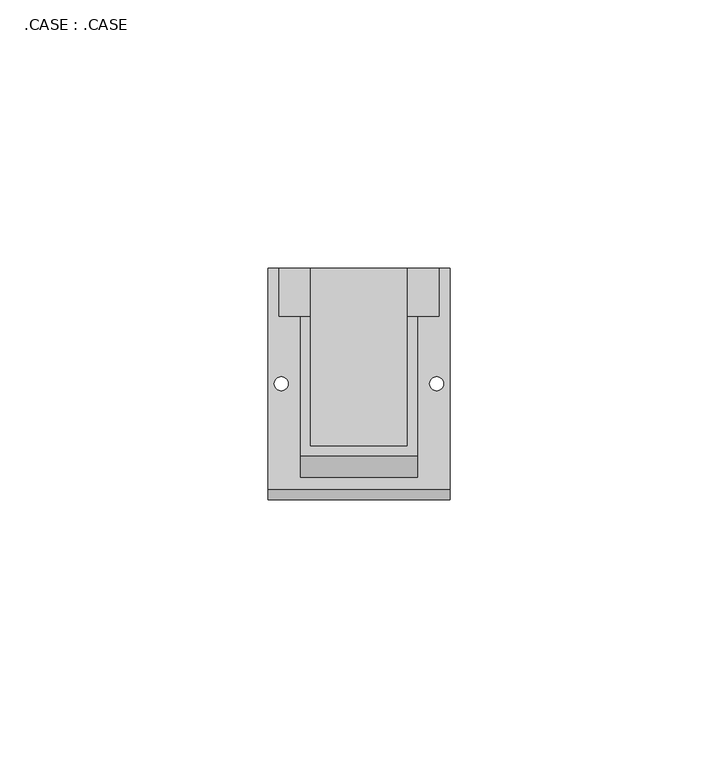
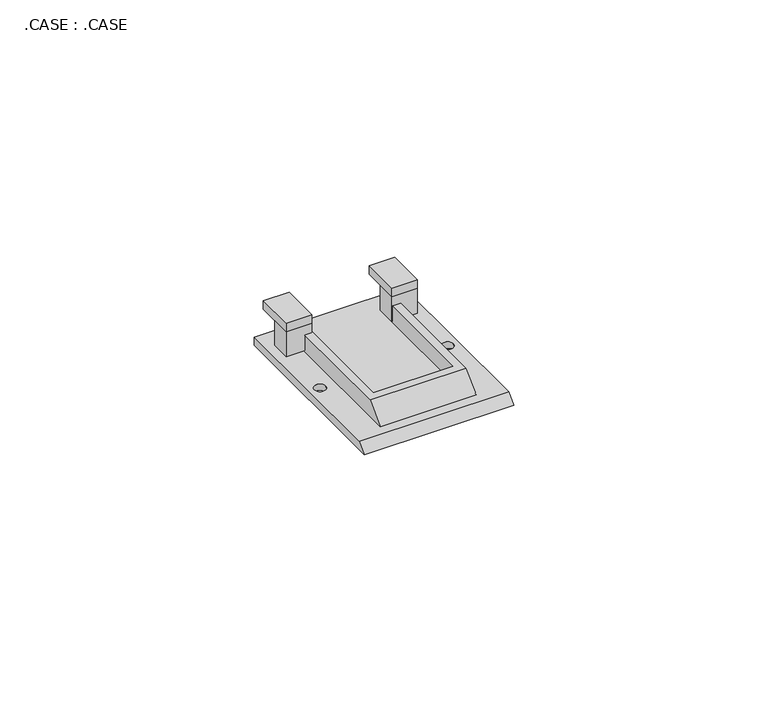
"""IFC4 building model written with IfcOpenShell, lengths in millimetres: proxy geometry, .CASE : .CASE."""

from ifc_helpers import new_model, si_unit, frame, origin, place, context, project, spatial, polyline, circle_curve, outline, extrude, source, transform, mapped, element, save
from ifc_brep_helpers import plane_surface, revolved_surface, advanced_brep


def case_case_fa127987(model_context):
    return source(origin(), model_context, "Body", "SolidModel", [
        extrude(outline(polyline([(1442.9350176, 13234.6739696), (1442.9350176, 13225.7186096), (1437.1350176, 13225.7186096), (1437.1350176, 13234.6739696), (1442.9350176, 13234.6739696)])), frame((0.0, 0.0, 8.0), z_axis=(0.0, 0.0, 1.0), x_axis=(1.0, 0.0, 0.0)), (0.0, 0.0, 1.0), 2.0),
        extrude(outline(polyline([(1461.1150176, 13234.6739696), (1466.9150176, 13234.6739696), (1466.9150176, 13225.7186096), (1461.1150176, 13225.7186096), (1461.1150176, 13234.6739696)])), frame((0.0, 0.0, 8.0), z_axis=(0.0, 0.0, 1.0), x_axis=(1.0, 0.0, 0.0)), (0.0, 0.0, 1.0), 2.0),
        extrude(outline(polyline([(1442.9350176, 13230.2186096), (1442.9350176, 13225.7186096), (1437.1350176, 13225.7186096), (1437.1350176, 13230.2186096), (1442.9350176, 13230.2186096)])), frame((0.0, 0.0, 2.0), z_axis=(0.0, 0.0, 1.0), x_axis=(1.0, 0.0, 0.0)), (0.0, 0.0, 1.0), 6.0),
        extrude(outline(polyline([(1461.1150176, 13230.2186096), (1466.9150176, 13230.2186096), (1466.9150176, 13225.7186096), (1461.1150176, 13225.7186096), (1461.1150176, 13230.2186096)])), frame((0.0, 0.0, 2.0), z_axis=(0.0, 0.0, 1.0), x_axis=(1.0, 0.0, 0.0)), (0.0, 0.0, 1.0), 6.0),
        advanced_brep(
        [(1469.0250176, 13193.4256546, 2.0), (1469.0250176, 13234.6739696, 2.0), (1435.0250176, 13234.6739696, 2.0), (1435.0250176, 13193.4256546, 2.0), (1441.1350176, 13195.6739696, 2.0), (1441.1350176, 13225.7186096, 2.0), (1442.9350176, 13225.7186096, 2.0), (1442.9350176, 13201.4739696, 2.0), (1461.1150176, 13201.4739696, 2.0), (1461.1150176, 13225.7186096, 2.0), (1462.9150176, 13225.7186096, 2.0), (1462.9150176, 13195.6739696, 2.0), (1467.8250176, 13213.1041412, 2.0), (1465.2250176, 13213.1041412, 2.0), (1438.8250176, 13213.1041412, 2.0), (1436.2250176, 13213.1041412, 2.0), (1435.0250176, 13234.6739696, 0.0), (1469.0250176, 13234.6739696, 0.0), (1469.0250176, 13191.4256546, 0.0), (1435.0250176, 13191.4256546, 0.0), (1464.5250176, 13213.1041412, 0.0), (1468.5250176, 13213.1041412, 0.0), (1435.5250176, 13213.1041412, 0.0), (1439.5250176, 13213.1041412, 0.0), (1441.1350176, 13225.7186096, 6.0), (1441.1350176, 13199.6739696, 6.0), (1462.9150176, 13199.6739696, 6.0), (1462.9150176, 13225.7186096, 6.0), (1461.1150176, 13225.7186096, 6.0), (1461.1150176, 13201.4739696, 6.0), (1442.9350176, 13201.4739696, 6.0), (1442.9350176, 13225.7186096, 6.0)],
        [
            (0, 1),
            (1, 2),
            (2, 3),
            (3, 0),
            (4, 5),
            (5, 6),
            (6, 7),
            (7, 8),
            (8, 9),
            (9, 10),
            (10, 11),
            (11, 4),
            (12, 13, circle_curve(frame((1466.5250176, 13213.1041412, 2.0), z_axis=(0.0, 0.0, -1.0), x_axis=(-1.0, 0.0, 0.0)), 1.3)),
            (13, 12, circle_curve(frame((1466.5250176, 13213.1041412, 2.0), z_axis=(0.0, 0.0, -1.0), x_axis=(1.0, 0.0, 0.0)), 1.3)),
            (14, 15, circle_curve(frame((1437.5250176, 13213.1041412, 2.0), z_axis=(0.0, 0.0, -1.0), x_axis=(-1.0, 0.0, 0.0)), 1.3)),
            (15, 14, circle_curve(frame((1437.5250176, 13213.1041412, 2.0), z_axis=(0.0, 0.0, -1.0), x_axis=(1.0, 0.0, 0.0)), 1.3)),
            (16, 17),
            (17, 18),
            (18, 19),
            (19, 16),
            (20, 21, circle_curve(frame((1466.5250176, 13213.1041412, 0.0), z_axis=(0.0, 0.0, 1.0), x_axis=(-1.0, 0.0, 0.0)), 2.0)),
            (21, 20, circle_curve(frame((1466.5250176, 13213.1041412, 0.0), z_axis=(0.0, 0.0, 1.0), x_axis=(1.0, 0.0, 0.0)), 2.0)),
            (22, 23, circle_curve(frame((1437.5250176, 13213.1041412, 0.0), z_axis=(0.0, 0.0, 1.0), x_axis=(-1.0, 0.0, 0.0)), 2.0)),
            (23, 22, circle_curve(frame((1437.5250176, 13213.1041412, 0.0), z_axis=(0.0, 0.0, 1.0), x_axis=(1.0, 0.0, 0.0)), 2.0)),
            (0, 18),
            (17, 1),
            (16, 2),
            (19, 3),
            (24, 25),
            (25, 26),
            (26, 27),
            (27, 28),
            (28, 29),
            (29, 30),
            (30, 31),
            (31, 24),
            (24, 5),
            (4, 25),
            (26, 11),
            (10, 27),
            (9, 28),
            (8, 29),
            (7, 30),
            (6, 31),
            (20, 13),
            (12, 21),
            (22, 15),
            (14, 23),
        ],
        [
            plane_surface(frame((1467.7850176, 13193.4256546, 2.0), z_axis=(0.0, 0.0, 1.0), x_axis=(1.0, 0.0, 0.0))),
            plane_surface(frame((1467.7850176, 13193.4256546, 0.0), z_axis=(0.0, 0.0, -1.0), x_axis=(-1.0, 0.0, 0.0))),
            plane_surface(frame((1469.0250176, 13193.4256546, 2.0), z_axis=(1.0, 0.0, 0.0), x_axis=(0.0, 0.0, -1.0))),
            plane_surface(frame((1469.0250176, 13234.6739696, 2.0), z_axis=(0.0, 1.0, 0.0), x_axis=(0.0, 0.0, -1.0))),
            plane_surface(frame((1435.0250176, 13234.6739696, 2.0), z_axis=(-1.0, 0.0, 0.0), x_axis=(0.0, 0.0, -1.0))),
            plane_surface(frame((1441.1350176, 13234.6739696, 6.0), z_axis=(0.0, 0.0, 1.0), x_axis=(0.0, -1.0, 0.0))),
            plane_surface(frame((1441.1350176, 13225.7186096, 6.0), z_axis=(-1.0, 0.0, 0.0), x_axis=(0.0, 0.0, -1.0))),
            plane_surface(frame((1462.9150176, 13199.6739696, 6.0), z_axis=(1.0, 0.0, 0.0), x_axis=(0.0, 0.0, -1.0))),
            plane_surface(frame((1462.9150176, 13225.7186096, 6.0), z_axis=(0.0, 1.0, 0.0), x_axis=(0.0, 0.0, -1.0))),
            plane_surface(frame((1461.1150176, 13225.7186096, 6.0), z_axis=(-1.0, 0.0, 0.0), x_axis=(0.0, 0.0, -1.0))),
            plane_surface(frame((1461.1150176, 13201.4739696, 6.0), z_axis=(0.0, 1.0, 0.0), x_axis=(0.0, 0.0, -1.0))),
            plane_surface(frame((1442.9350176, 13201.4739696, 6.0), z_axis=(1.0, 0.0, 0.0), x_axis=(0.0, 0.0, -1.0))),
            plane_surface(frame((1442.9350176, 13225.7186096, 6.0), z_axis=(0.0, 1.0, 0.0), x_axis=(0.0, 0.0, -1.0))),
            plane_surface(frame((1441.1350176, 13195.6739696, 2.0), z_axis=(0.0, -0.7071067811865885, 0.7071067811865066), x_axis=(1.0, 0.0, 0.0))),
            revolved_surface(polyline([(1464.5250176, 13213.1041412, 0.0), (1465.2250176017499, 13213.1041412, 2.0)]), (1466.5250176, 13213.1041412, 5.7142857), (0.0, 0.0, -1.0)),
            revolved_surface(polyline([(1435.5250176, 13213.1041412, 0.0), (1436.2250176017499, 13213.1041412, 2.0)]), (1437.5250176, 13213.1041412, 5.7142857), (0.0, 0.0, -1.0)),
            plane_surface(frame((1435.0250176, 13191.4256546, 0.0), z_axis=(0.0, -0.707106781186628, 0.7071067811864672), x_axis=(1.0, 0.0, 0.0))),
        ],
        [
            (0, [[1, 2, 3, 4], [5, 6, 7, 8, 9, 10, 11, 12], [13, 14], [15, 16]]),
            (1, [[17, 18, 19, 20], [21, 22], [23, 24]]),
            (2, [[-1, 25, -18, 26]]),
            (3, [[-2, -26, -17, 27]]),
            (4, [[-3, -27, -20, 28]]),
            (5, [[29, 30, 31, 32, 33, 34, 35, 36]]),
            (6, [[-29, 37, -5, 38]]),
            (7, [[-31, 39, -11, 40]]),
            (8, [[-32, -40, -10, 41]]),
            (9, [[-33, -41, -9, 42]]),
            (10, [[-34, -42, -8, 43]]),
            (11, [[-35, -43, -7, 44]]),
            (12, [[-36, -44, -6, -37]]),
            (13, [[-38, -12, -39, -30]]),
            (14, [[45, -13, 46, -21]]),
            (14, [[-45, -22, -46, -14]]),
            (15, [[47, -15, 48, -23]]),
            (15, [[-47, -24, -48, -16]]),
            (16, [[-28, -19, -25, -4]]),
        ],
    ),
    ])


if __name__ == "__main__":
    model = new_model("IFC4")
    model_context = context("Model", 3, world=origin())
    ifc_project = project(units=[si_unit("LENGTHUNIT", "METRE", prefix="MILLI")], contexts=[model_context])
    site = spatial("IfcSite", under=ifc_project)
    building = spatial("IfcBuilding", under=site)
    placement = place(None, origin())
    case_case_shape = case_case_fa127987(model_context)
    element("IfcBuildingElementProxy", 1, Name=".CASE : .CASE", ObjectType=".CASE : .CASE", at=placement, inside=building, context=model_context, shape_type="MappedRepresentation", body=[
        mapped(case_case_shape, transform((0.0, 0.0, 0.0), x_axis=(1.0, 0.0, 0.0), y_axis=(0.0, 1.0, 0.0), z_axis=(0.0, 0.0, 1.0))),
    ])
    save(model, "model.ifc")

# Revit data of these elements
# Element 1 (IfcBuildingElementProxy, ".CASE : .CASE")
#   Materials on its faces: "Areia"
# Materials
#   "Areia": class "Genérico", colour RGB 191 183 178, transparency 0, Description = "Areia", Cost = 0
